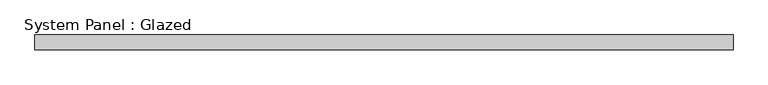
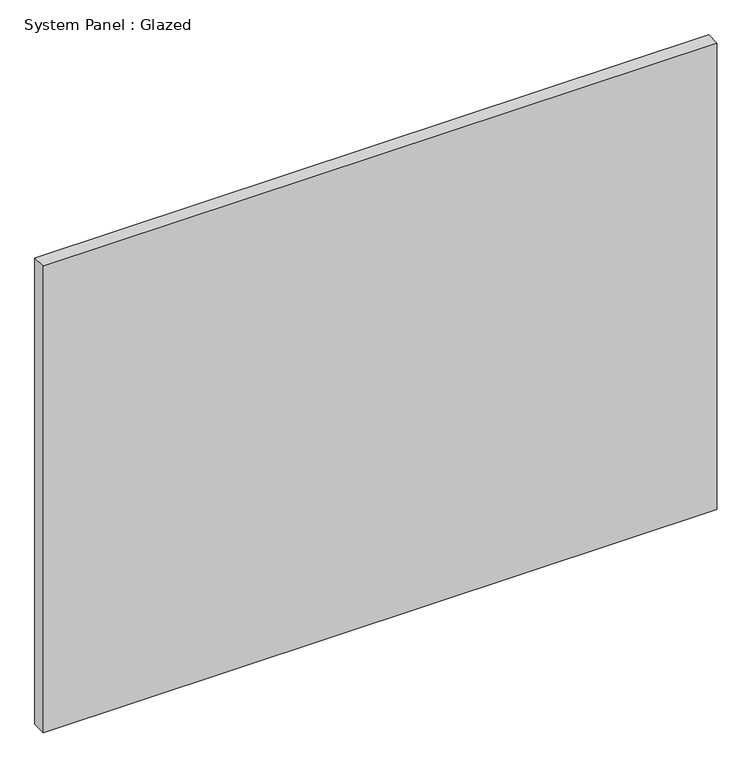
"""IFC4 building model written with IfcOpenShell, lengths in millimetres: plate geometry, System Panel : Glazed."""

from ifc_helpers import new_model, si_unit, origin, origin_with_axes, place, context, project, spatial, polyline, outline, extrude, source, transform, mapped, element, save


def system_panel_glazed_8a7cc684(model_context):
    return source(origin(), model_context, "Body", "SweptSolid", [
        extrude(outline(polyline([(594.4075643, 19.05), (-594.4075643, 19.05), (-594.4075643, 44.45), (594.4075643, 44.45), (594.4075643, 19.05)])), origin_with_axes(), (0.0, 0.0, 1.0), 869.95),
    ])


if __name__ == "__main__":
    model = new_model("IFC4")
    model_context = context("Model", 3, world=origin())
    ifc_project = project(units=[si_unit("LENGTHUNIT", "METRE", prefix="MILLI")], contexts=[model_context])
    site = spatial("IfcSite", under=ifc_project)
    building = spatial("IfcBuilding", under=site)
    placement = place(None, origin())
    system_panel_glazed_shape = system_panel_glazed_8a7cc684(model_context)
    element("IfcPlate", 1, ObjectType="System Panel : Glazed", at=placement, inside=building, context=model_context, shape_type="MappedRepresentation", body=[
        mapped(system_panel_glazed_shape, transform((0.0, 0.0, 0.0), x_axis=(1.0, 0.0, 0.0), y_axis=(0.0, 1.0, 0.0), z_axis=(0.0, 0.0, 1.0))),
    ])
    save(model, "model.ifc")

# Revit data of these elements
# Element 1 (IfcPlate, "System Panel : Glazed")
#   Materials on its faces: "Glass"
# Materials
#   "Glass": class "Glass", colour RGB 0 128 192, transparency 0.75
